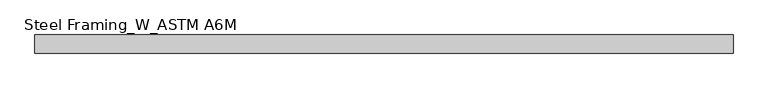
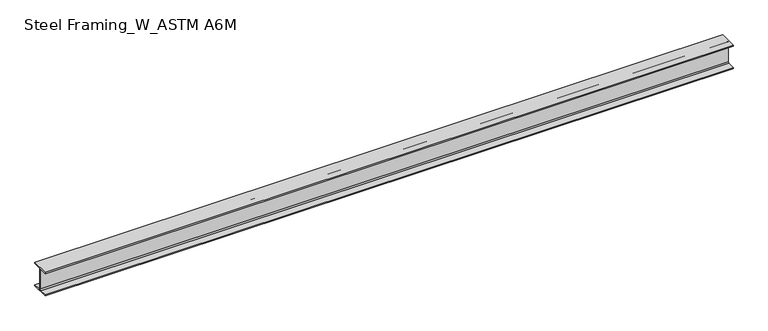
"""IFC4 building model written with IfcOpenShell, lengths in millimetres: beam geometry, Steel Framing_W_ASTM A6M : H_SB_AR_S02_W360x91_B3."""

import ifcopenshell
import ifcopenshell.guid

model = None  # the IFC model being written
_history = None  # IfcOwnerHistory: only IFC2X3 demands one
_inside = {}  # id of a spatial element -> (the spatial element, [elements in it])
_under = {}  # id of a project, library or spatial element -> (it, [spatial elements below it])
_declared = {}  # id of a project -> (the project, [libraries it declares])
_typed = {}  # id of a type object -> (the type object, [elements of that type])
_made_of = {}  # id of a material, layer set ... -> (it, [elements and type objects made of it])


def new_model(schema):
    """Start an empty IFC model of exactly this schema.

    Asked for "IFC4X3", IfcOpenShell would pick the latest addendum, in which some entities
    have other attributes; the version numbers below select the first issue.
    IFC2X3 requires an IfcOwnerHistory on every rooted entity: one is made here for all.
    """
    global model, _history
    if schema == "IFC4X3":
        model = ifcopenshell.file(schema_version=(4, 3, 0, 0))
    else:
        model = ifcopenshell.file(schema=schema)
    _inside.clear()
    _under.clear()
    _declared.clear()
    _typed.clear()
    _made_of.clear()
    _history = None
    if model.schema == "IFC2X3":
        org = make("IfcOrganization", Name="unknown")
        user = make(
            "IfcPersonAndOrganization",
            ThePerson=make("IfcPerson", FamilyName="unknown"),
            TheOrganization=org,
        )
        app = make(
            "IfcApplication",
            ApplicationDeveloper=org,
            Version="unknown",
            ApplicationFullName="unknown",
            ApplicationIdentifier="unknown",
        )
        _history = make(
            "IfcOwnerHistory",
            OwningUser=user,
            OwningApplication=app,
            ChangeAction="ADDED",
            CreationDate=0,
        )
    return model


def make(cls, **values):
    """One entity of the class cls with the attributes given. An attribute that is None is left unset."""
    return model.create_entity(
        cls, **{name: value for name, value in values.items() if value is not None}
    )


def rooted(cls, **values):
    """An entity with a GlobalId (a new one), such as an element, a storey or a relation."""
    return make(cls, GlobalId=ifcopenshell.guid.new(), OwnerHistory=_history, **values)


def si_unit(unit_type, name, prefix=None):
    """IfcSIUnit, for example si_unit("LENGTHUNIT", "METRE", prefix="MILLI")."""
    return make("IfcSIUnit", UnitType=unit_type, Prefix=prefix, Name=name)


def assignment(units):
    """IfcUnitAssignment: the units of a project."""
    return None if units is None else make("IfcUnitAssignment", Units=units)


def point(xyz):
    """IfcCartesianPoint."""
    return None if xyz is None else make("IfcCartesianPoint", Coordinates=xyz)


def direction(xyz):
    """IfcDirection."""
    return None if xyz is None else make("IfcDirection", DirectionRatios=xyz)


def frame(location, z_axis=None, x_axis=None):
    """IfcAxis2Placement3D, a coordinate frame: its origin and axes. An axis left out is left unset."""
    return make(
        "IfcAxis2Placement3D",
        Location=point(location),
        Axis=direction(z_axis),
        RefDirection=direction(x_axis),
    )


def frame_2d(location, x_axis=None):
    """IfcAxis2Placement2D, a coordinate frame in the plane: its origin and x axis."""
    return make(
        "IfcAxis2Placement2D", Location=point(location), RefDirection=direction(x_axis)
    )


def origin():
    """The frame at (0, 0, 0) with its axes left unset."""
    return frame((0.0, 0.0, 0.0))


def place(relative_to, where):
    """IfcLocalPlacement: puts the frame where relative to a parent placement (None: the world)."""
    return make(
        "IfcLocalPlacement", PlacementRelTo=relative_to, RelativePlacement=where
    )


def context(
    kind, dimensions, precision=None, world=None, true_north=None, identifier=None
):
    """IfcGeometricRepresentationContext, for example the 3D "Model" context."""
    return make(
        "IfcGeometricRepresentationContext",
        ContextIdentifier=identifier,
        ContextType=kind,
        CoordinateSpaceDimension=dimensions,
        Precision=precision,
        WorldCoordinateSystem=world,
        TrueNorth=true_north,
    )


def project(units=None, contexts=None):
    """IfcProject with its units and contexts."""
    return rooted(
        "IfcProject",
        Name="project",
        RepresentationContexts=contexts,
        UnitsInContext=assignment(units),
    )


def spatial(cls, under=None, at=None, **own):
    """A site, building, storey or space (cls), placed at a placement, below another one or the project."""
    s = rooted(cls, ObjectPlacement=at, **own)
    if under is not None:
        _under.setdefault(under.id(), (under, []))[1].append(s)
    return s


def polyline(points):
    """IfcPolyline through the points."""
    return make("IfcPolyline", Points=[point(p) for p in points])


def circle_curve(where, radius):
    """IfcCircle in the frame where."""
    return make("IfcCircle", Position=where, Radius=radius)


def trimmed(basis, trim1, trim2, sense, master):
    """IfcTrimmedCurve: the piece of a basis curve between two trims."""
    return make(
        "IfcTrimmedCurve",
        BasisCurve=basis,
        Trim1=trim1,
        Trim2=trim2,
        SenseAgreement=sense,
        MasterRepresentation=master,
    )


def segment(curve, same_sense, transition):
    """IfcCompositeCurveSegment."""
    return make(
        "IfcCompositeCurveSegment",
        Transition=transition,
        SameSense=same_sense,
        ParentCurve=curve,
    )


def composite_curve(segments, self_intersect=None):
    """IfcCompositeCurve: segments joined end to end."""
    return make("IfcCompositeCurve", Segments=segments, SelfIntersect=self_intersect)


def outline(outer, holes=None, kind="AREA"):
    """IfcArbitraryClosedProfileDef: a profile drawn as a closed curve; with holes, ...WithVoids."""
    if holes is None:
        return make("IfcArbitraryClosedProfileDef", ProfileType=kind, OuterCurve=outer)
    return make(
        "IfcArbitraryProfileDefWithVoids",
        ProfileType=kind,
        OuterCurve=outer,
        InnerCurves=holes,
    )


def extrude(swept, where, along, depth):
    """IfcExtrudedAreaSolid: the profile swept, set in the frame where, extruded along a direction by depth."""
    return make(
        "IfcExtrudedAreaSolid",
        SweptArea=swept,
        Position=where,
        ExtrudedDirection=direction(along),
        Depth=depth,
    )


def shape(context_of_items, identifier, shape_type, items):
    """IfcShapeRepresentation: the items that make up one representation, for example the "Body"."""
    return make(
        "IfcShapeRepresentation",
        ContextOfItems=context_of_items,
        RepresentationIdentifier=identifier,
        RepresentationType=shape_type,
        Items=items,
    )


def source(mapping_origin, context_of_items, identifier, shape_type, items):
    """IfcRepresentationMap: a shape defined once, which mapped items show again and again."""
    return make(
        "IfcRepresentationMap",
        MappingOrigin=mapping_origin,
        MappedRepresentation=shape(context_of_items, identifier, shape_type, items),
    )


def transform(
    local_origin,
    x_axis=None,
    y_axis=None,
    z_axis=None,
    scale=None,
    scale2=None,
    scale3=None,
    uniform=True,
):
    """IfcCartesianTransformationOperator3D, or its non-uniform kind. x_axis, y_axis, z_axis: its Axis1, 2, 3."""
    if uniform:
        return make(
            "IfcCartesianTransformationOperator3D",
            Axis1=direction(x_axis),
            Axis2=direction(y_axis),
            LocalOrigin=point(local_origin),
            Scale=scale,
            Axis3=direction(z_axis),
        )
    return make(
        "IfcCartesianTransformationOperator3DnonUniform",
        Axis1=direction(x_axis),
        Axis2=direction(y_axis),
        LocalOrigin=point(local_origin),
        Scale=scale,
        Axis3=direction(z_axis),
        Scale2=scale2,
        Scale3=scale3,
    )


def mapped(mapping_source, mapping_target):
    """IfcMappedItem: shows the shape of a source again, moved by a transform."""
    return make(
        "IfcMappedItem", MappingSource=mapping_source, MappingTarget=mapping_target
    )


def made_of(thing, what):
    """Note that an element or type object is made of a material, layer set ...; save() writes the relation."""
    if what is not None:
        _made_of.setdefault(what.id(), (what, []))[1].append(thing)
    return thing


def element(
    cls,
    number,
    at=None,
    inside=None,
    cuts=None,
    type_object=None,
    material=None,
    context=None,
    identifier="Body",
    shape_type=None,
    held_by="IfcProductDefinitionShape",
    body=None,
    shapes=None,
    **own,
):
    """One element of the class cls, such as IfcWall. Its Tag is "e" and its number.

    at: its placement. inside: the storey or other place that contains it. cuts: it is an
    opening in that element (IfcRelVoidsElement). A single representation is given by context,
    identifier, shape_type and body (its items); several are given by shapes. held_by: the class
    of the entity that holds the representations. save() writes the other relations.
    """
    e = rooted(cls, Tag="e%d" % number, ObjectPlacement=at, **own)
    if body is not None:
        shapes = [shape(context, identifier, shape_type, body)]
    if shapes is not None:
        e.Representation = make(held_by, Representations=shapes)
    if inside is not None:
        _inside.setdefault(inside.id(), (inside, []))[1].append(e)
    if cuts is not None:
        rooted(
            "IfcRelVoidsElement", RelatingBuildingElement=cuts, RelatedOpeningElement=e
        )
    if type_object is not None:
        _typed.setdefault(type_object.id(), (type_object, []))[1].append(e)
    return made_of(e, material)


def aggregate(whole, parts):
    """IfcRelAggregates: a whole, such as a stair, and the parts it consists of."""
    return rooted("IfcRelAggregates", RelatingObject=whole, RelatedObjects=parts)


def save(model, path):
    """Write the relations noted so far, then the file.

    IfcRelAggregates (storeys below a building ...), IfcRelContainedInSpatialStructure (elements
    in a storey), IfcRelDefinesByType, IfcRelAssociatesMaterial and IfcRelDeclares: one each for
    every whole, place, type object, material and project.
    """
    for whole, parts in _under.values():
        aggregate(whole, parts)
    for where, things in _inside.values():
        rooted(
            "IfcRelContainedInSpatialStructure",
            RelatedElements=things,
            RelatingStructure=where,
        )
    for kind, things in _typed.values():
        rooted("IfcRelDefinesByType", RelatedObjects=things, RelatingType=kind)
    for what, things in _made_of.values():
        rooted("IfcRelAssociatesMaterial", RelatedObjects=things, RelatingMaterial=what)
    for by, libraries in _declared.values():
        rooted("IfcRelDeclares", RelatingContext=by, RelatedDefinitions=libraries)
    model.write(path)


def steel_framing_w_astm_a6m_37bec3ec(model_context):
    return source(origin(), model_context, "Body", "SweptSolid", [
        extrude(outline(composite_curve([segment(polyline([(127.0, -160.1), (127.0, -176.5), (-127.0, -176.5), (-127.0, -160.1), (-19.865, -160.1)]), True, "CONTINUOUS"), segment(trimmed(circle_curve(frame_2d((-19.865, -145.0)), 15.1), [point((-19.865, -160.1))], [point((-4.765, -145.0))], True, "CARTESIAN"), True, "CONTINUOUS"), segment(polyline([(-4.765, -145.0), (-4.765, 145.0)]), True, "CONTINUOUS"), segment(trimmed(circle_curve(frame_2d((-19.865, 145.0)), 15.1), [point((-4.765, 145.0))], [point((-19.865, 160.1))], True, "CARTESIAN"), True, "CONTINUOUS"), segment(polyline([(-19.865, 160.1), (-127.0, 160.1), (-127.0, 176.5), (127.0, 176.5), (127.0, 160.1), (19.865, 160.1)]), True, "CONTINUOUS"), segment(trimmed(circle_curve(frame_2d((19.865, 145.0)), 15.1), [point((19.865, 160.1))], [point((4.765, 145.0))], True, "CARTESIAN"), True, "CONTINUOUS"), segment(polyline([(4.765, 145.0), (4.765, -145.0)]), True, "CONTINUOUS"), segment(trimmed(circle_curve(frame_2d((19.865, -145.0)), 15.1), [point((4.765, -145.0))], [point((19.865, -160.1))], True, "CARTESIAN"), True, "CONTINUOUS"), segment(polyline([(19.865, -160.1), (127.0, -160.1)]), True, "CONTINUOUS")], self_intersect=False)), frame((-4885.8, 0.0, 0.0), z_axis=(1.0, 0.0, 0.0), x_axis=(0.0, 1.0, 0.0)), (0.0, 0.0, 1.0), 9771.6),
    ])


if __name__ == "__main__":
    model = new_model("IFC4")
    model_context = context("Model", 3, world=origin())
    ifc_project = project(units=[si_unit("LENGTHUNIT", "METRE", prefix="MILLI")], contexts=[model_context])
    site = spatial("IfcSite", under=ifc_project)
    building = spatial("IfcBuilding", under=site)
    placement = place(None, origin())
    steel_framing_w_astm_a6m_shape = steel_framing_w_astm_a6m_37bec3ec(model_context)
    element("IfcBeam", 1, ObjectType="Steel Framing_W_ASTM A6M : H_SB_AR_S02_W360x91_B3", at=placement, inside=building, context=model_context, shape_type="MappedRepresentation", body=[
        mapped(steel_framing_w_astm_a6m_shape, transform((0.0, 0.0, 0.0), x_axis=(1.0, 0.0, 0.0), y_axis=(0.0, 1.0, 0.0), z_axis=(0.0, 0.0, 1.0))),
    ])
    save(model, "model.ifc")

# Revit data of these elements
# Type "Steel Framing_W_ASTM A6M : H_SB_AR_S02_W360x91_B3"
#   Type Mark = "B3"
#   Section Name Key = "W14x61"
#   Width = 25.4 cm
#   Web Thickness = 0.953 cm
#   Web Fillet = 1.51 cm
#   Warping Constant = 1260000.0 cm⁶
#   Torsional Moment of Inertia = 91.20 cm⁴
#   Section Area = 115.0 cm²
#   Plastic Modulus weak axis = 537.0 cm³
#   Plastic Modulus strong axis = 1670.0 cm³
#   Perimeter = 1.68 m²/m
#   Nominal Weight = 91.00 kgf/m
#   Moment of Inertia weak axis = 4450.00 cm⁴
#   Moment of Inertia strong axis = 26600.00 cm⁴
#   Height = 35.3 cm
#   Flange Thickness = 1.64 cm
#   Elastic Modulus weak axis = 352.0 cm³
#   Elastic Modulus strong axis = 1510.0 cm³
#   Centroid Vertical = 17.65 cm
#   Centroid Horizontal = 12.7 cm
#   Length [instance default] = 1500 mm
#   Structural Material [instance default] = Steel, 45-345
#   Bolt Spacing = 0
#   Assembly Code = ""
# Element 1 (IfcBeam, "Steel Framing_W_ASTM A6M : H_SB_AR_S02_W360x91_B3")
#   Materials on its faces: "Steel, 45-345"
# Materials
#   "Steel, 45-345": class "Metal", colour RGB 189 187 185, transparency 0, Description = "Steel 345 MPa", Cost = 0
